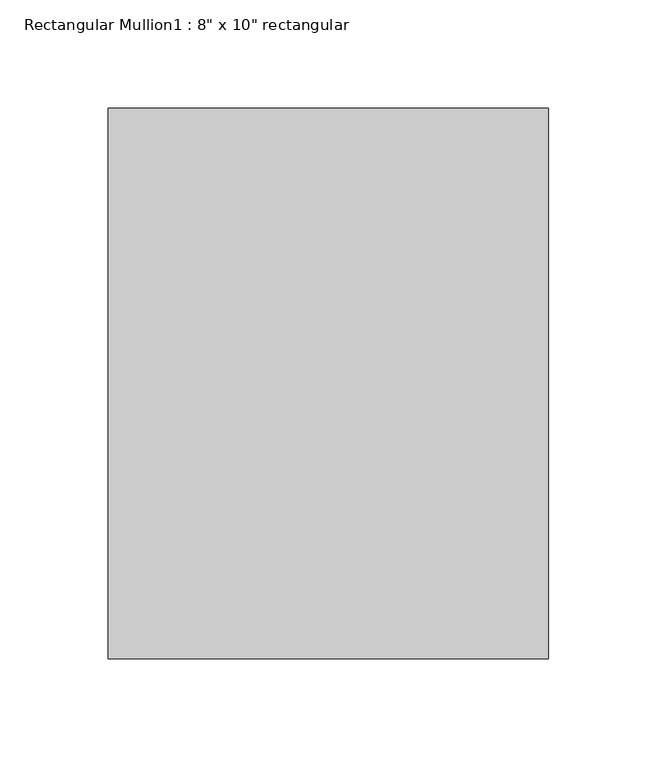
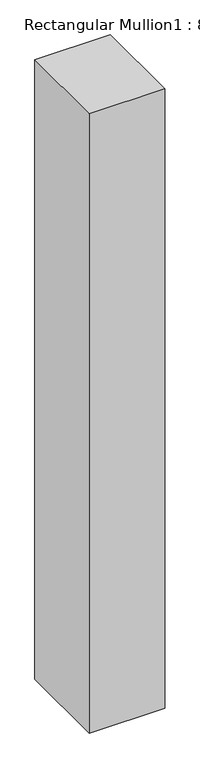
"""IFC4 building model written with IfcOpenShell, lengths in millimetres: member geometry."""

from ifc_helpers import new_model, si_unit, frame, origin, place, context, project, spatial, polyline, outline, extrude, source, transform, mapped, element, save


def member_707c4438(model_context):
    return source(origin(), model_context, "Body", "SweptSolid", [
        extrude(outline(polyline([(101.6, 127.0), (101.6, -127.0), (-101.6, -127.0), (-101.6, 127.0), (101.6, 127.0)])), frame((0.0, 0.0, -1765.3), z_axis=(0.0, 0.0, 1.0), x_axis=(1.0, 0.0, 0.0)), (0.0, 0.0, 1.0), 1765.3),
    ])


if __name__ == "__main__":
    model = new_model("IFC4")
    model_context = context("Model", 3, world=origin())
    ifc_project = project(units=[si_unit("LENGTHUNIT", "METRE", prefix="MILLI")], contexts=[model_context])
    site = spatial("IfcSite", under=ifc_project)
    building = spatial("IfcBuilding", under=site)
    placement = place(None, origin())
    member_shape = member_707c4438(model_context)
    element("IfcMember", 1, ObjectType="Rectangular Mullion1 : 8\" x 10\" rectangular", at=placement, inside=building, context=model_context, shape_type="MappedRepresentation", body=[
        mapped(member_shape, transform((0.0, 0.0, 0.0), x_axis=(1.0, 0.0, 0.0), y_axis=(0.0, 1.0, 0.0), z_axis=(0.0, 0.0, 1.0))),
    ])
    save(model, "model.ifc")

# Revit data of these elements
# Type "Rectangular Mullion1 : 8\" x 10\" rectangular"
#   built-in parameter 1007304 = 0.833333 (stored number, unit not read)
#   built-in parameter 1007301 = 0.333333 (stored number, unit not read)
#   built-in parameter 1007300 = 0.333333 (stored number, unit not read)
# Element 1 (IfcMember, "Rectangular Mullion1 : 8\" x 10\" rectangular")
#   Materials on its faces: "support-frame"
# Materials
#   "support-frame": class "Unassigned", colour RGB 233 233 233, transparency 0, Cost = 0
